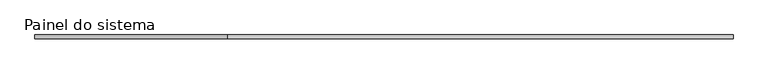
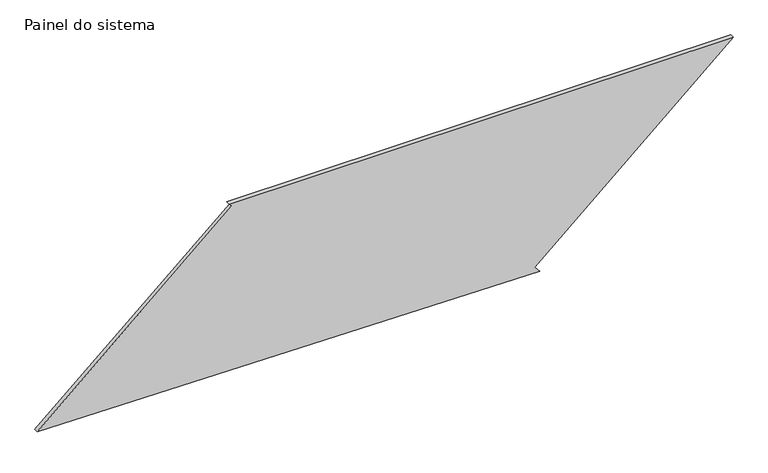
"""IFC4 building model written with IfcOpenShell, lengths in millimetres: plate geometry, Painel do sistema : Envidraçado."""

from ifc_helpers import new_model, si_unit, frame, origin, place, context, project, spatial, polyline, outline, extrude, source, transform, mapped, element, save


def painel_do_sistema_09091d53(model_context):
    return source(origin(), model_context, "Body", "SweptSolid", [
        extrude(outline(polyline([(0.0, 972.0375502), (37.6158083, 939.0974383), (1130.9740408, 2187.6528115), (1130.9740408, -979.9977782), (1112.1661367, -963.5277223), (40.2014704, -2187.6528115), (0.0, 972.0375502)])), frame((0.0, 24.5, 0.0), z_axis=(0.0, 1.0, 0.0), x_axis=(0.0, 0.0, 1.0)), (0.0, 0.0, 1.0), 25.0),
    ])


if __name__ == "__main__":
    model = new_model("IFC4")
    model_context = context("Model", 3, world=origin())
    ifc_project = project(units=[si_unit("LENGTHUNIT", "METRE", prefix="MILLI")], contexts=[model_context])
    site = spatial("IfcSite", under=ifc_project)
    building = spatial("IfcBuilding", under=site)
    placement = place(None, origin())
    painel_do_sistema_shape = painel_do_sistema_09091d53(model_context)
    element("IfcPlate", 1, ObjectType="Painel do sistema : Envidraçado", at=placement, inside=building, context=model_context, shape_type="MappedRepresentation", body=[
        mapped(painel_do_sistema_shape, transform((0.0, 0.0, 0.0), x_axis=(1.0, 0.0, 0.0), y_axis=(0.0, 1.0, 0.0), z_axis=(0.0, 0.0, 1.0))),
    ])
    save(model, "model.ifc")

# Revit data of these elements
# Type "Painel do sistema : Envidraçado"
#   Construction Type Id = "GSP4R"
#   Analytic Construction = "Vidraça única Pilkington 1/8 pol"
#   Visual Light Transmittance = 0.9
#   Solar Heat Gain Coefficient = 0.86
#   Heat Transfer Coefficient (U) = 6.7069 W/(m²·K)
# Element 1 (IfcPlate, "Painel do sistema : Envidraçado")
#   Materials on its faces: "Vidro"
# Materials
#   "Vidro": class "Vidro", colour RGB 0 128 192, transparency 0.9, Description = "Vidro de sílica", Cost = 0
